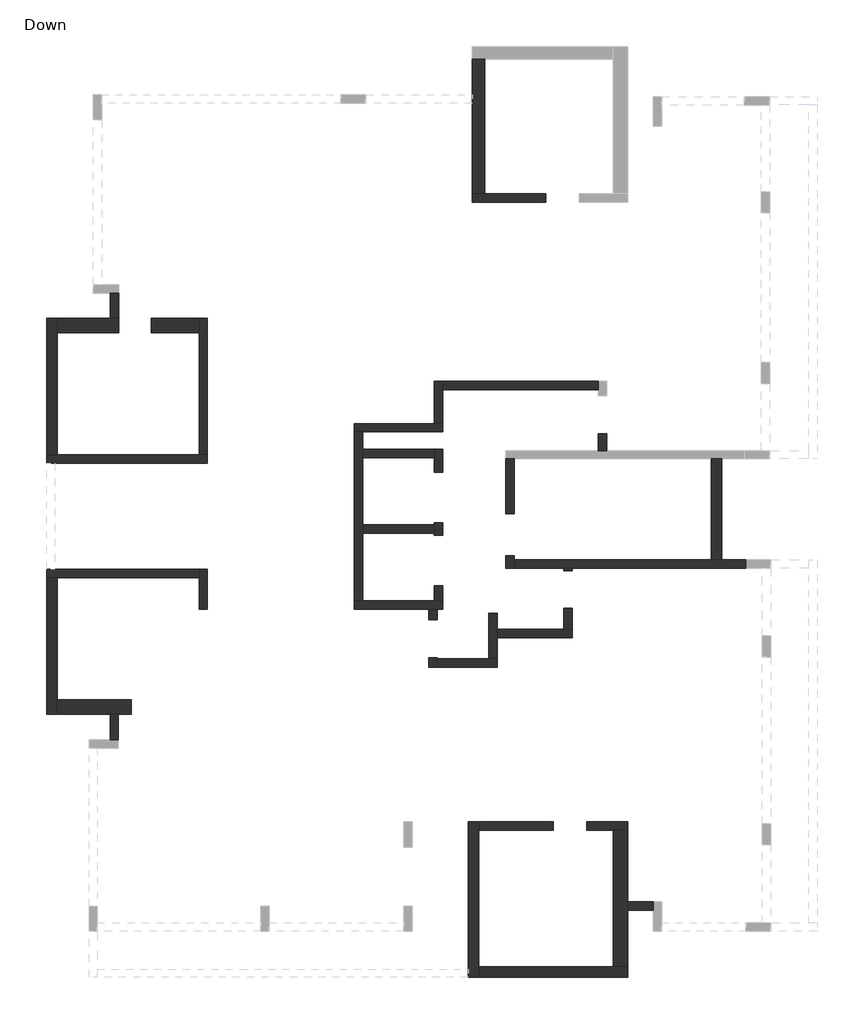
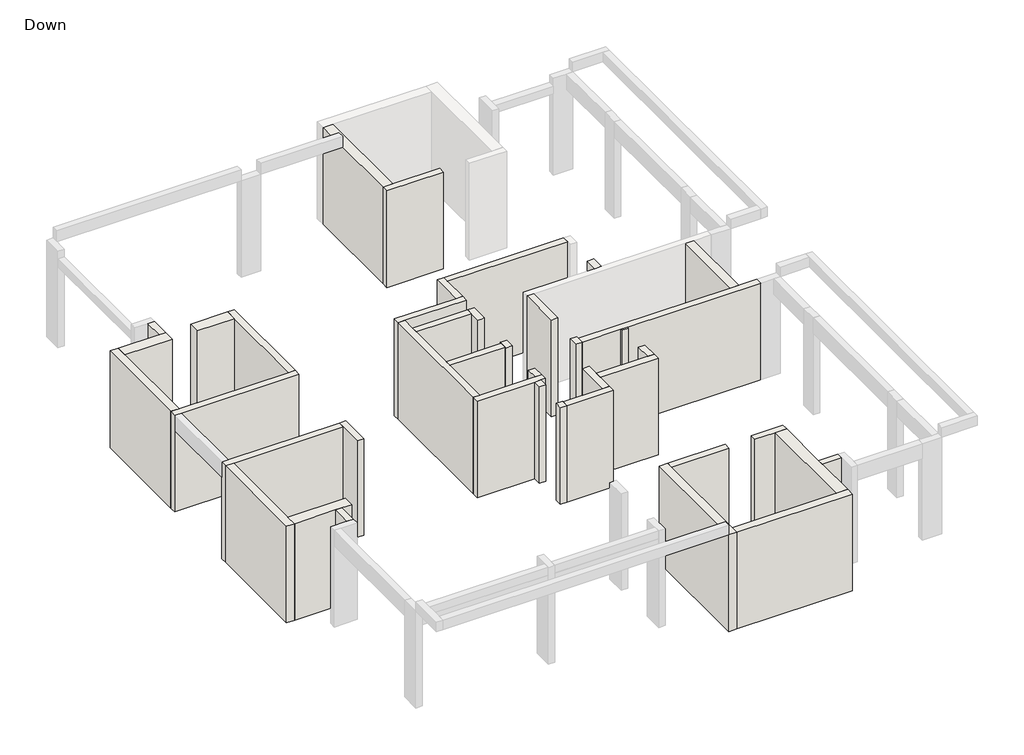
# One storey, part 1 of 2: 41 walls.
"""IFC4 building model written with IfcOpenShell, lengths in millimetres."""

from ifc_helpers import new_model, si_unit, origin, origin_with_axes, place, context, project, spatial, polyline, outline, extrude, faceted_brep, element, save

model = new_model("IFC4")

# Units and contexts
model_context = context("Model", 3, world=origin())
ifc_project = project(units=[si_unit("LENGTHUNIT", "METRE", prefix="MILLI")], contexts=[model_context])

# Site, building, storey
site = spatial("IfcSite", under=ifc_project)
building = spatial("IfcBuilding", under=site)
storey = spatial("IfcBuildingStorey", under=building, Name="Down", Elevation=0.0)

# Walls
placement = place(None, origin())
element("IfcWall", 1, ObjectType="20", at=placement, inside=storey, context=model_context, shape_type="Brep", body=[
    faceted_brep([(-7842.7593383, -3416.4704639, 0.0), (-7842.7593383, -2465.8036059, 0.0), (-7842.7593383, -2465.8036059, 2900.0), (-7842.7593383, -2465.8036059, 3150.0), (-7842.7593383, -3416.4704639, 3150.0), (-7842.7593383, -3416.4704639, 2900.0), (-8042.7593383, -3416.4704639, 0.0), (-8042.7593383, -3416.4704639, 2900.0), (-8042.7593383, -3416.4704639, 3150.0), (-8042.7593383, -2665.8036059, 3150.0), (-8042.7593383, -2465.8036059, 3150.0), (-8042.7593383, -2465.8036059, 0.0), (-8042.7593383, -2665.8036059, 0.0)], [[[0, 1, 2, 3, 4, 5]], [[6, 7, 8, 9, 10, 11, 12]], [[1, 0, 6, 12, 11]], [[4, 3, 10, 9, 8]], [[0, 5, 4, 8, 7, 6]], [[3, 2, 1, 11, 10]]]),
])
element("IfcWall", 2, ObjectType="20", at=placement, inside=storey, context=model_context, shape_type="Brep", body=[
    faceted_brep([(-8042.7593383, -2465.8036059, 0.0), (-11667.5737279, -2465.8036059, 0.0), (-11667.5737279, -2465.8036059, 3150.0), (-11467.5737279, -2465.8036059, 3150.0), (-8042.7593383, -2465.8036059, 3150.0), (-8042.7593383, -2665.8036059, 0.0), (-8042.7593383, -2665.8036059, 2900.0), (-8042.7593383, -2665.8036059, 3150.0), (-11417.5737279, -2665.8036059, 3150.0), (-11667.5737279, -2665.8036059, 3150.0), (-11667.5737279, -2665.8036059, 0.0), (-11417.5737279, -2665.8036059, 0.0)], [[[0, 1, 2, 3, 4]], [[5, 6, 7, 8, 9, 10, 11]], [[1, 0, 5, 11, 10]], [[4, 3, 2, 9, 8, 7]], [[0, 4, 7, 6, 5]], [[2, 1, 10, 9]]]),
])
element("IfcWall", 3, ObjectType="20", at=placement, inside=storey, context=model_context, shape_type="Brep", body=[
    faceted_brep([(-10157.6225223, -5916.9995493, 0.0), (-10157.6225223, -6521.9995493, 0.0), (-10157.6225223, -6521.9995493, 3150.0), (-10157.6225223, -5916.9995493, 3150.0), (-9957.6225223, -5916.9995493, 0.0), (-9957.6225223, -5916.9995493, 2900.0), (-9957.6225223, -5916.9995493, 3150.0), (-9957.6225223, -6521.9995493, 3150.0), (-9957.6225223, -6521.9995493, 0.0)], [[[0, 1, 2, 3]], [[4, 5, 6, 7, 8]], [[1, 0, 4, 8]], [[2, 1, 8, 7]], [[3, 2, 7, 6]], [[0, 3, 6, 5, 4]]]),
])
element("IfcWall", 4, ObjectType="20", at=placement, inside=storey, context=model_context, shape_type="Brep", body=[
    faceted_brep([(-11667.5737279, 47.4292682, 0.0), (-7841.6160164, 47.4292682, 0.0), (-7841.6160164, 47.4292682, 2900.0), (-7841.6160164, 47.4292682, 3150.0), (-11467.5737279, 47.4292682, 3150.0), (-11667.5737279, 47.4292682, 3150.0), (-11667.5737279, 247.4292682, 0.0), (-11667.5737279, 247.4292682, 3150.0), (-11417.5737279, 247.4292682, 3150.0), (-8041.6160164, 247.4292682, 3150.0), (-7841.6160164, 247.4292682, 3150.0), (-7841.6160164, 247.4292682, 0.0), (-8041.6160164, 247.4292682, 0.0), (-11417.5737279, 247.4292682, 0.0)], [[[0, 1, 2, 3, 4, 5]], [[6, 7, 8, 9, 10, 11, 12, 13]], [[1, 0, 6, 13, 12, 11]], [[5, 4, 3, 10, 9, 8, 7]], [[3, 2, 1, 11, 10]], [[0, 5, 7, 6]]]),
])
element("IfcWall", 5, ObjectType="20", at=placement, inside=storey, context=model_context, shape_type="Brep", body=[
    faceted_brep([(-7841.6160164, 247.4292682, 0.0), (-7841.6160164, 3498.6252115, 0.0), (-7841.6160164, 3498.6252115, 2900.0), (-7841.6160164, 3498.6252115, 3150.0), (-7841.6160164, 247.4292682, 3150.0), (-8041.6160164, 247.4292682, 0.0), (-8041.6160164, 247.4292682, 2900.0), (-8041.6160164, 247.4292682, 3150.0), (-8041.6160164, 3148.6252115, 3150.0), (-8041.6160164, 3498.6252115, 3150.0), (-8041.6160164, 3498.6252115, 0.0), (-8041.6160164, 3148.6252115, 0.0)], [[[0, 1, 2, 3, 4]], [[5, 6, 7, 8, 9, 10, 11]], [[1, 0, 5, 11, 10]], [[4, 3, 9, 8, 7]], [[0, 4, 7, 6, 5]], [[3, 2, 1, 10, 9]]]),
])
element("IfcWall", 6, ObjectType="20", at=placement, inside=storey, context=model_context, shape_type="Brep", body=[
    faceted_brep([(-4348.0741106, -3416.4704639, 0.0), (-2578.9868545, -3416.4704639, 0.0), (-2378.9868545, -3416.4704639, 0.0), (-2247.7143708, -3416.4704639, 0.0), (-2247.7143708, -3416.4704639, 2900.0), (-2247.7143708, -3416.4704639, 3150.0), (-2378.9868545, -3416.4704639, 3150.0), (-2578.9868545, -3416.4704639, 3150.0), (-4348.0741106, -3416.4704639, 3150.0), (-4348.0741106, -3416.4704639, 2900.0), (-4348.0741106, -3216.4704639, 0.0), (-4348.0741106, -3216.4704639, 3150.0), (-4148.0741106, -3216.4704639, 3150.0), (-2447.7143708, -3216.4704639, 3150.0), (-2247.7143708, -3216.4704639, 3150.0), (-2247.7143708, -3216.4704639, 0.0), (-2447.7143708, -3216.4704639, 0.0), (-4148.0741106, -3216.4704639, 0.0)], [[[0, 1, 2, 3, 4, 5, 6, 7, 8, 9]], [[10, 11, 12, 13, 14, 15, 16, 17]], [[3, 2, 1, 0, 10, 17, 16, 15]], [[8, 7, 6, 5, 14, 13, 12, 11]], [[5, 4, 3, 15, 14]], [[0, 9, 8, 11, 10]]]),
])
element("IfcWall", 7, ObjectType="20", at=placement, inside=storey, context=model_context, shape_type="Brep", body=[
    faceted_brep([(-2247.7143708, -3216.4704639, 0.0), (-2247.7143708, -2865.9729515, 0.0), (-2247.7143708, -2865.9729515, 2900.0), (-2247.7143708, -2865.9729515, 3150.0), (-2247.7143708, -3216.4704639, 3150.0), (-2447.7143708, -3216.4704639, 0.0), (-2447.7143708, -3216.4704639, 3150.0), (-2447.7143708, -2865.9729515, 3150.0), (-2447.7143708, -2865.9729515, 0.0), (-2347.7143708, -2865.9729515, 3150.0)], [[[0, 1, 2, 3, 4]], [[5, 6, 7, 8]], [[1, 0, 5, 8]], [[3, 2, 1, 8, 7, 9]], [[4, 3, 9, 7, 6]], [[0, 4, 6, 5]]]),
])
element("IfcWall", 8, ObjectType="20", at=placement, inside=storey, context=model_context, shape_type="Brep", body=[
    faceted_brep([(-2247.7143708, -1665.4649148, 0.0), (-2247.7143708, -1366.9258792, 0.0), (-2247.7143708, -1366.9258792, 2900.0), (-2247.7143708, -1366.9258792, 3150.0), (-2247.7143708, -1665.4649148, 3150.0), (-2247.7143708, -1665.4649148, 2900.0), (-2447.7143708, -1665.4649148, 0.0), (-2447.7143708, -1665.4649148, 3150.0), (-2447.7143708, -1616.7670579, 3150.0), (-2447.7143708, -1416.7670579, 3150.0), (-2447.7143708, -1366.9258792, 3150.0), (-2447.7143708, -1366.9258792, 0.0), (-2447.7143708, -1416.7670579, 0.0), (-2447.7143708, -1616.7670579, 0.0), (-2347.7143708, -1366.9258792, 3150.0), (-2347.7143708, -1665.4649148, 3150.0)], [[[0, 1, 2, 3, 4, 5]], [[6, 7, 8, 9, 10, 11, 12, 13]], [[1, 0, 6, 13, 12, 11]], [[3, 2, 1, 11, 10, 14]], [[4, 3, 14, 10, 9, 8, 7, 15]], [[0, 5, 4, 15, 7, 6]]]),
])
element("IfcWall", 9, ObjectType="20", at=placement, inside=storey, context=model_context, shape_type="SweptSolid", body=[
    extrude(outline(polyline([(-4148.0741106, -1416.7670579), (-2447.7143708, -1416.7670579), (-2447.7143708, -1616.7670579), (-4148.0741106, -1616.7670579), (-4148.0741106, -1416.7670579)])), origin_with_axes(), (0.0, 0.0, 1.0), 3150.0),
])
element("IfcWall", 10, ObjectType="20", at=placement, inside=storey, context=model_context, shape_type="Brep", body=[
    faceted_brep([(-4348.0741106, 794.07967, 0.0), (-4348.0741106, -3216.4704639, 0.0), (-4348.0741106, -3216.4704639, 3150.0), (-4348.0741106, 47.4292682, 3150.0), (-4348.0741106, 794.07967, 3150.0), (-4148.0741106, 794.07967, 0.0), (-4148.0741106, 794.07967, 2900.0), (-4148.0741106, 794.07967, 3150.0), (-4148.0741106, 384.07967, 3150.0), (-4148.0741106, 184.07967, 3150.0), (-4148.0741106, -1416.7670579, 3150.0), (-4148.0741106, -1616.7670579, 3150.0), (-4148.0741106, -3216.4704639, 3150.0), (-4148.0741106, -3216.4704639, 0.0), (-4148.0741106, -1616.7670579, 0.0), (-4148.0741106, -1416.7670579, 0.0), (-4148.0741106, 184.07967, 0.0), (-4148.0741106, 384.07967, 0.0)], [[[0, 1, 2, 3, 4]], [[5, 6, 7, 8, 9, 10, 11, 12, 13, 14, 15, 16, 17]], [[1, 0, 5, 17, 16, 15, 14, 13]], [[4, 3, 2, 12, 11, 10, 9, 8, 7]], [[2, 1, 13, 12]], [[0, 4, 7, 6, 5]]]),
])
element("IfcWall", 11, ObjectType="20", at=placement, inside=storey, context=model_context, shape_type="Brep", body=[
    faceted_brep([(-2247.7143708, -166.4178424, 0.0), (-2247.7143708, 384.07967, 0.0), (-2247.7143708, 384.07967, 2900.0), (-2247.7143708, 384.07967, 3150.0), (-2247.7143708, -166.4178424, 3150.0), (-2247.7143708, -166.4178424, 2900.0), (-2447.7143708, -166.4178424, 0.0), (-2447.7143708, -166.4178424, 3150.0), (-2447.7143708, 184.07967, 3150.0), (-2447.7143708, 384.07967, 3150.0), (-2447.7143708, 384.07967, 0.0), (-2447.7143708, 184.07967, 0.0), (-2347.7143708, -166.4178424, 3150.0)], [[[0, 1, 2, 3, 4, 5]], [[6, 7, 8, 9, 10, 11]], [[1, 0, 6, 11, 10]], [[4, 3, 9, 8, 7, 12]], [[0, 5, 4, 12, 7, 6]], [[3, 2, 1, 10, 9]]]),
])
element("IfcWall", 12, ObjectType="20", at=placement, inside=storey, context=model_context, shape_type="Brep", body=[
    faceted_brep([(-2447.7143708, 384.07967, 0.0), (-4148.0741106, 384.07967, 0.0), (-4148.0741106, 384.07967, 2900.0), (-4148.0741106, 384.07967, 3150.0), (-2447.7143708, 384.07967, 3150.0), (-2447.7143708, 184.07967, 0.0), (-2447.7143708, 184.07967, 3150.0), (-4148.0741106, 184.07967, 3150.0), (-4148.0741106, 184.07967, 0.0)], [[[0, 1, 2, 3, 4]], [[5, 6, 7, 8]], [[1, 0, 5, 8]], [[4, 3, 7, 6]], [[0, 4, 6, 5]], [[3, 2, 1, 8, 7]]]),
])
element("IfcWall", 13, ObjectType="20", at=placement, inside=storey, context=model_context, shape_type="Brep", body=[
    faceted_brep([(-4348.0741106, 794.07967, 0.0), (-4148.0741106, 794.07967, 0.0), (-2249.8316689, 794.07967, 0.0), (-2249.8316689, 794.07967, 2900.0), (-2249.8316689, 794.07967, 3150.0), (-4148.0741106, 794.07967, 3150.0), (-4348.0741106, 794.07967, 3150.0), (-4348.0741106, 994.07967, 0.0), (-4348.0741106, 994.07967, 2900.0), (-4348.0741106, 994.07967, 3150.0), (-2449.8316689, 994.07967, 3150.0), (-2249.8316689, 994.07967, 3150.0), (-2249.8316689, 994.07967, 0.0), (-2449.8316689, 994.07967, 0.0)], [[[0, 1, 2, 3, 4, 5, 6]], [[7, 8, 9, 10, 11, 12, 13]], [[2, 1, 0, 7, 13, 12]], [[6, 5, 4, 11, 10, 9]], [[4, 3, 2, 12, 11]], [[0, 6, 9, 8, 7]]]),
])
element("IfcWall", 14, ObjectType="20", at=placement, inside=storey, context=model_context, shape_type="Brep", body=[
    faceted_brep([(-2249.8316689, 994.07967, 0.0), (-2249.8316689, 1803.8127355, 0.0), (-2249.8316689, 2003.8127355, 0.0), (-2249.8316689, 2003.8127355, 3150.0), (-2249.8316689, 1803.8127355, 3150.0), (-2249.8316689, 994.07967, 3150.0), (-2449.8316689, 994.07967, 0.0), (-2449.8316689, 994.07967, 2900.0), (-2449.8316689, 994.07967, 3150.0), (-2449.8316689, 2003.8127355, 3150.0), (-2449.8316689, 2003.8127355, 2900.0), (-2449.8316689, 2003.8127355, 0.0)], [[[0, 1, 2, 3, 4, 5]], [[6, 7, 8, 9, 10, 11]], [[2, 1, 0, 6, 11]], [[5, 4, 3, 9, 8]], [[0, 5, 8, 7, 6]], [[3, 2, 11, 10, 9]]]),
])
element("IfcWall", 15, ObjectType="20", at=placement, inside=storey, context=model_context, shape_type="Brep", body=[
    faceted_brep([(-2249.8316689, 1803.8127355, 0.0), (1452.348775, 1803.8127355, 0.0), (1452.348775, 1803.8127355, 2900.0), (1452.348775, 1803.8127355, 3150.0), (-2249.8316689, 1803.8127355, 3150.0), (-2249.8316689, 1803.8127355, 2900.0), (-2249.8316689, 2003.8127355, 0.0), (-2249.8316689, 2003.8127355, 3150.0), (1452.348775, 2003.8127355, 3150.0), (1452.348775, 2003.8127355, 0.0)], [[[0, 1, 2, 3, 4, 5]], [[6, 7, 8, 9]], [[1, 0, 6, 9]], [[4, 3, 8, 7]], [[0, 5, 4, 7, 6]], [[3, 2, 1, 9, 8]]]),
])
element("IfcWall", 16, ObjectType="20", at=placement, inside=storey, context=model_context, shape_type="Brep", body=[
    faceted_brep([(1452.348775, 750.3722456, 0.0), (1452.348775, 352.3201981, 0.0), (1452.348775, 352.3201981, 2900.0), (1452.348775, 352.3201981, 3150.0), (1452.348775, 750.3722456, 3150.0), (1452.348775, 750.3722456, 2900.0), (1652.348775, 750.3722456, 0.0), (1652.348775, 750.3722456, 2900.0), (1652.348775, 750.3722456, 3150.0), (1652.348775, 352.3201981, 3150.0), (1652.348775, 352.3201981, 2900.0), (1652.348775, 352.3201981, 0.0), (1552.348775, 750.3722456, 3150.0)], [[[0, 1, 2, 3, 4, 5]], [[6, 7, 8, 9, 10, 11]], [[1, 0, 6, 11]], [[4, 3, 9, 8, 12]], [[0, 5, 4, 12, 8, 7, 6]], [[3, 2, 1, 11, 10, 9]]]),
])
element("IfcWall", 17, ObjectType="20", at=placement, inside=storey, context=model_context, shape_type="Brep", body=[
    faceted_brep([(-748.6672985, 152.3201981, 0.0), (-748.6672985, -1148.8441723, 0.0), (-748.6672985, -1148.8441723, 2900.0), (-748.6672985, -1148.8441723, 3150.0), (-748.6672985, 152.3201981, 3150.0), (-548.6672985, 152.3201981, 0.0), (-548.6672985, 152.3201981, 3150.0), (-548.6672985, -1148.8441723, 3150.0), (-548.6672985, -1148.8441723, 2900.0), (-548.6672985, -1148.8441723, 0.0)], [[[0, 1, 2, 3, 4]], [[5, 6, 7, 8, 9]], [[1, 0, 5, 9]], [[3, 2, 1, 9, 8, 7]], [[4, 3, 7, 6]], [[0, 4, 6, 5]]]),
])
element("IfcWall", 18, ObjectType="20", at=placement, inside=storey, context=model_context, shape_type="Brep", body=[
    faceted_brep([(-748.6672985, -2148.2088872, 0.0), (-748.6672985, -2446.7479228, 0.0), (-748.6672985, -2446.7479228, 2900.0), (-748.6672985, -2446.7479228, 3150.0), (-748.6672985, -2148.2088872, 3150.0), (-748.6672985, -2148.2088872, 2900.0), (-548.6672985, -2148.2088872, 0.0), (-548.6672985, -2148.2088872, 2900.0), (-548.6672985, -2148.2088872, 3150.0), (-548.6672985, -2246.7479228, 3150.0), (-548.6672985, -2446.7479228, 3150.0), (-548.6672985, -2446.7479228, 0.0), (-548.6672985, -2246.7479228, 0.0)], [[[0, 1, 2, 3, 4, 5]], [[6, 7, 8, 9, 10, 11, 12]], [[1, 0, 6, 12, 11]], [[4, 3, 10, 9, 8]], [[0, 5, 4, 8, 7, 6]], [[3, 2, 1, 11, 10]]]),
])
element("IfcWall", 19, ObjectType="20", at=placement, inside=storey, context=model_context, shape_type="Brep", body=[
    faceted_brep([(-548.6672985, -2446.7479228, 0.0), (633.928377, -2446.7479228, 0.0), (833.928377, -2446.7479228, 0.0), (4951.7310336, -2446.7479228, 0.0), (4951.7310336, -2446.7479228, 3150.0), (833.928377, -2446.7479228, 3150.0), (633.928377, -2446.7479228, 3150.0), (-548.6672985, -2446.7479228, 3150.0), (-548.6672985, -2246.7479228, 0.0), (-548.6672985, -2246.7479228, 3150.0), (4133.663356, -2246.7479228, 3150.0), (4383.663356, -2246.7479228, 3150.0), (4951.7310336, -2246.7479228, 3150.0), (4951.7310336, -2246.7479228, 0.0), (4383.663356, -2246.7479228, 0.0), (4133.663356, -2246.7479228, 0.0)], [[[0, 1, 2, 3, 4, 5, 6, 7]], [[8, 9, 10, 11, 12, 13, 14, 15]], [[3, 2, 1, 0, 8, 15, 14, 13]], [[4, 3, 13, 12]], [[7, 6, 5, 4, 12, 11, 10, 9]], [[0, 7, 9, 8]]]),
])
element("IfcWall", 20, ObjectType="20", at=placement, inside=storey, context=model_context, shape_type="Brep", body=[
    faceted_brep([(-1396.4017034, -8672.5783859, 0.0), (379.852602, -8672.5783859, 0.0), (379.852602, -8672.5783859, 2900.0), (379.852602, -8672.5783859, 3150.0), (-1396.4017034, -8672.5783859, 3150.0), (-1396.4017034, -8672.5783859, 2900.0), (-1396.4017034, -8472.5783859, 0.0), (-1396.4017034, -8472.5783859, 3150.0), (379.852602, -8472.5783859, 3150.0), (379.852602, -8472.5783859, 2900.0), (379.852602, -8472.5783859, 0.0)], [[[0, 1, 2, 3, 4, 5]], [[6, 7, 8, 9, 10]], [[1, 0, 6, 10]], [[3, 2, 1, 10, 9, 8]], [[4, 3, 8, 7]], [[0, 5, 4, 7, 6]]]),
])
element("IfcWall", 21, ObjectType="20", at=placement, inside=storey, context=model_context, shape_type="Brep", body=[
    faceted_brep([(1180.1912932, -8672.5783859, 0.0), (1805.1912932, -8672.5783859, 0.0), (2155.1912932, -8672.5783859, 0.0), (2155.1912932, -8672.5783859, 3150.0), (1805.1912932, -8672.5783859, 3150.0), (1180.1912932, -8672.5783859, 3150.0), (1180.1912932, -8672.5783859, 2900.0), (1180.1912932, -8472.5783859, 0.0), (1180.1912932, -8472.5783859, 2900.0), (1180.1912932, -8472.5783859, 3150.0), (2155.1912932, -8472.5783859, 3150.0), (2155.1912932, -8472.5783859, 2900.0), (2155.1912932, -8472.5783859, 0.0)], [[[0, 1, 2, 3, 4, 5, 6]], [[7, 8, 9, 10, 11, 12]], [[2, 1, 0, 7, 12]], [[5, 4, 3, 10, 9]], [[0, 6, 5, 9, 8, 7]], [[3, 2, 12, 11, 10]]]),
])
element("IfcWall", 22, ObjectType="20", at=placement, inside=storey, context=model_context, shape_type="Brep", body=[
    faceted_brep([(2753.3437999, -10374.7377812, 0.0), (2155.1912932, -10374.7377812, 0.0), (2155.1912932, -10374.7377812, 2900.0), (2155.1912932, -10374.7377812, 3150.0), (2753.3437999, -10374.7377812, 3150.0), (2753.3437999, -10574.7377812, 0.0), (2753.3437999, -10574.7377812, 3150.0), (2155.1912932, -10574.7377812, 3150.0), (2155.1912932, -10574.7377812, 0.0)], [[[0, 1, 2, 3, 4]], [[5, 6, 7, 8]], [[1, 0, 5, 8]], [[4, 3, 7, 6]], [[0, 4, 6, 5]], [[3, 2, 1, 8, 7]]]),
])
element("IfcWall", 23, ObjectType="20", at=placement, inside=storey, context=model_context, shape_type="Brep", body=[
    faceted_brep([(-2578.9868545, -3416.4704639, 0.0), (-2578.9868545, -3670.5462389, 0.0), (-2578.9868545, -3670.5462389, 2900.0), (-2578.9868545, -3670.5462389, 3150.0), (-2578.9868545, -3416.4704639, 3150.0), (-2578.9868545, -3416.4704639, 2900.0), (-2378.9868545, -3416.4704639, 0.0), (-2378.9868545, -3416.4704639, 2900.0), (-2378.9868545, -3416.4704639, 3150.0), (-2378.9868545, -3670.5462389, 3150.0), (-2378.9868545, -3670.5462389, 2900.0), (-2378.9868545, -3670.5462389, 0.0)], [[[0, 1, 2, 3, 4, 5]], [[6, 7, 8, 9, 10, 11]], [[1, 0, 6, 11]], [[3, 2, 1, 11, 10, 9]], [[4, 3, 9, 8]], [[0, 5, 4, 8, 7, 6]]]),
])
element("IfcWall", 24, ObjectType="20", at=placement, inside=storey, context=model_context, shape_type="Brep", body=[
    faceted_brep([(-2578.9868545, -4570.3979419, 0.0), (-2578.9868545, -4796.9488413, 0.0), (-2578.9868545, -4796.9488413, 2900.0), (-2578.9868545, -4796.9488413, 3150.0), (-2578.9868545, -4570.3979419, 3150.0), (-2578.9868545, -4570.3979419, 2900.0), (-2378.9868545, -4570.3979419, 0.0), (-2378.9868545, -4570.3979419, 2900.0), (-2378.9868545, -4570.3979419, 3150.0), (-2378.9868545, -4596.9488413, 3150.0), (-2378.9868545, -4796.9488413, 3150.0), (-2378.9868545, -4796.9488413, 0.0), (-2378.9868545, -4596.9488413, 0.0)], [[[0, 1, 2, 3, 4, 5]], [[6, 7, 8, 9, 10, 11, 12]], [[1, 0, 6, 12, 11]], [[4, 3, 10, 9, 8]], [[0, 5, 4, 8, 7, 6]], [[3, 2, 1, 11, 10]]]),
])
element("IfcWall", 25, ObjectType="20", at=placement, inside=storey, context=model_context, shape_type="Brep", body=[
    faceted_brep([(-2378.9868545, -4796.9488413, 0.0), (-951.9279184, -4796.9488413, 0.0), (-951.9279184, -4796.9488413, 2900.0), (-951.9279184, -4796.9488413, 3150.0), (-2378.9868545, -4796.9488413, 3150.0), (-2378.9868545, -4596.9488413, 0.0), (-2378.9868545, -4596.9488413, 2900.0), (-2378.9868545, -4596.9488413, 3150.0), (-1151.9279184, -4596.9488413, 3150.0), (-951.9279184, -4596.9488413, 3150.0), (-951.9279184, -4596.9488413, 0.0), (-1151.9279184, -4596.9488413, 0.0)], [[[0, 1, 2, 3, 4]], [[5, 6, 7, 8, 9, 10, 11]], [[1, 0, 5, 11, 10]], [[4, 3, 9, 8, 7]], [[0, 4, 7, 6, 5]], [[3, 2, 1, 10, 9]]]),
])
element("IfcWall", 26, ObjectType="20", at=placement, inside=storey, context=model_context, shape_type="Brep", body=[
    faceted_brep([(-951.9279184, -4596.9488413, 0.0), (-951.9279184, -4098.2404601, 0.0), (-951.9279184, -3898.2404601, 0.0), (-951.9279184, -3515.9834758, 0.0), (-951.9279184, -3515.9834758, 2900.0), (-951.9279184, -3515.9834758, 3150.0), (-951.9279184, -3898.2404601, 3150.0), (-951.9279184, -4098.2404601, 3150.0), (-951.9279184, -4596.9488413, 3150.0), (-1151.9279184, -4596.9488413, 0.0), (-1151.9279184, -4596.9488413, 2900.0), (-1151.9279184, -4596.9488413, 3150.0), (-1151.9279184, -3515.9834758, 3150.0), (-1151.9279184, -3515.9834758, 2900.0), (-1151.9279184, -3515.9834758, 0.0)], [[[0, 1, 2, 3, 4, 5, 6, 7, 8]], [[9, 10, 11, 12, 13, 14]], [[3, 2, 1, 0, 9, 14]], [[5, 4, 3, 14, 13, 12]], [[8, 7, 6, 5, 12, 11]], [[0, 8, 11, 10, 9]]]),
])
element("IfcWall", 27, ObjectType="20", at=placement, inside=storey, context=model_context, shape_type="Brep", body=[
    faceted_brep([(-951.9279184, -4098.2404601, 0.0), (833.928377, -4098.2404601, 0.0), (833.928377, -4098.2404601, 2900.0), (833.928377, -4098.2404601, 3150.0), (-951.9279184, -4098.2404601, 3150.0), (-951.9279184, -4098.2404601, 2900.0), (-951.9279184, -3898.2404601, 0.0), (-951.9279184, -3898.2404601, 2900.0), (-951.9279184, -3898.2404601, 3150.0), (633.928377, -3898.2404601, 3150.0), (833.928377, -3898.2404601, 3150.0), (833.928377, -3898.2404601, 0.0), (633.928377, -3898.2404601, 0.0)], [[[0, 1, 2, 3, 4, 5]], [[6, 7, 8, 9, 10, 11, 12]], [[1, 0, 6, 12, 11]], [[4, 3, 10, 9, 8]], [[0, 5, 4, 8, 7, 6]], [[3, 2, 1, 11, 10]]]),
])
element("IfcWall", 28, ObjectType="20", at=placement, inside=storey, context=model_context, shape_type="Brep", body=[
    faceted_brep([(833.928377, -3898.2404601, 0.0), (833.928377, -3399.5320789, 0.0), (833.928377, -3399.5320789, 2900.0), (833.928377, -3399.5320789, 3150.0), (833.928377, -3898.2404601, 3150.0), (633.928377, -3898.2404601, 0.0), (633.928377, -3898.2404601, 2900.0), (633.928377, -3898.2404601, 3150.0), (633.928377, -3399.5320789, 3150.0), (633.928377, -3399.5320789, 2900.0), (633.928377, -3399.5320789, 0.0)], [[[0, 1, 2, 3, 4]], [[5, 6, 7, 8, 9, 10]], [[1, 0, 5, 10]], [[3, 2, 1, 10, 9, 8]], [[4, 3, 8, 7]], [[0, 4, 7, 6, 5]]]),
])
element("IfcWall", 29, ObjectType="20", at=placement, inside=storey, context=model_context, shape_type="Brep", body=[
    faceted_brep([(833.928377, -2499.6803759, 0.0), (833.928377, -2446.7479228, 0.0), (833.928377, -2446.7479228, 2900.0), (833.928377, -2446.7479228, 3150.0), (833.928377, -2499.6803759, 3150.0), (833.928377, -2499.6803759, 2900.0), (633.928377, -2499.6803759, 0.0), (633.928377, -2499.6803759, 2900.0), (633.928377, -2499.6803759, 3150.0), (633.928377, -2446.7479228, 3150.0), (633.928377, -2446.7479228, 2900.0), (633.928377, -2446.7479228, 0.0)], [[[0, 1, 2, 3, 4, 5]], [[6, 7, 8, 9, 10, 11]], [[1, 0, 6, 11]], [[4, 3, 9, 8]], [[0, 5, 4, 8, 7, 6]], [[3, 2, 1, 11, 10, 9]]]),
])
element("IfcWall", 30, ObjectType="20", at=placement, inside=storey, context=model_context, shape_type="Brep", body=[
    faceted_brep([(-1546.8886915, 6257.4646681, 0.0), (199.8822614, 6257.4646681, 0.0), (199.8822614, 6257.4646681, 2900.0), (199.8822614, 6257.4646681, 3150.0), (-1546.8886915, 6257.4646681, 3150.0), (-1546.8886915, 6257.4646681, 2900.0), (-1546.8886915, 6457.4646681, 0.0), (-1546.8886915, 6457.4646681, 3150.0), (-1246.8886915, 6457.4646681, 3150.0), (199.8822614, 6457.4646681, 3150.0), (199.8822614, 6457.4646681, 2900.0), (199.8822614, 6457.4646681, 0.0), (-1246.8886915, 6457.4646681, 0.0)], [[[0, 1, 2, 3, 4, 5]], [[6, 7, 8, 9, 10, 11, 12]], [[1, 0, 6, 12, 11]], [[3, 2, 1, 11, 10, 9]], [[4, 3, 9, 8, 7]], [[0, 5, 4, 7, 6]]]),
])
element("IfcWall", 31, ObjectType="20", at=placement, inside=storey, context=model_context, shape_type="SweptSolid", body=[
    extrude(outline(polyline([(-9955.8228668, 4097.8205808), (-9955.8228668, 3498.6252115), (-10155.8228668, 3498.6252115), (-10155.8228668, 4097.8205808), (-9955.8228668, 4097.8205808)])), origin_with_axes(), (0.0, 0.0, 1.0), 3150.0),
])
element("IfcWall", 32, ObjectType="25", at=placement, inside=storey, context=model_context, shape_type="Brep", body=[
    faceted_brep([(-11667.5737279, -2665.8036059, 0.0), (-11667.5737279, -5916.9995493, 0.0), (-11667.5737279, -5916.9995493, 3150.0), (-11667.5737279, -2665.8036059, 3150.0), (-11417.5737279, -2665.8036059, 0.0), (-11417.5737279, -2665.8036059, 2900.0), (-11417.5737279, -2665.8036059, 3150.0), (-11417.5737279, -5566.9995493, 3150.0), (-11417.5737279, -5916.9995493, 3150.0), (-11417.5737279, -5916.9995493, 0.0), (-11417.5737279, -5566.9995493, 0.0)], [[[0, 1, 2, 3]], [[4, 5, 6, 7, 8, 9, 10]], [[1, 0, 4, 10, 9]], [[3, 2, 8, 7, 6]], [[0, 3, 6, 5, 4]], [[2, 1, 9, 8]]]),
])
element("IfcWall", 33, ObjectType="25", at=placement, inside=storey, context=model_context, shape_type="Brep", body=[
    faceted_brep([(-11417.5737279, 247.4292682, 0.0), (-11417.5737279, 3148.6252115, 0.0), (-11417.5737279, 3498.6252115, 0.0), (-11417.5737279, 3498.6252115, 3150.0), (-11417.5737279, 3148.6252115, 3150.0), (-11417.5737279, 247.4292682, 3150.0), (-11417.5737279, 247.4292682, 2900.0), (-11667.5737279, 247.4292682, 0.0), (-11667.5737279, 247.4292682, 3150.0), (-11667.5737279, 3498.6252115, 3150.0), (-11667.5737279, 3498.6252115, 0.0)], [[[0, 1, 2, 3, 4, 5, 6]], [[7, 8, 9, 10]], [[2, 1, 0, 7, 10]], [[5, 4, 3, 9, 8]], [[3, 2, 10, 9]], [[0, 6, 5, 8, 7]]]),
])
element("IfcWall", 34, ObjectType="25", at=placement, inside=storey, context=model_context, shape_type="SweptSolid", body=[
    extrude(outline(polyline([(4383.663356, 152.3201981), (4383.663356, -2246.7479228), (4133.663356, -2246.7479228), (4133.663356, 152.3201981), (4383.663356, 152.3201981)])), origin_with_axes(), (0.0, 0.0, 1.0), 3150.0),
])
element("IfcWall", 35, ObjectType="25", at=placement, inside=storey, context=model_context, shape_type="Brep", body=[
    faceted_brep([(-1646.4017034, -8472.5783859, 0.0), (-1646.4017034, -12173.6155079, 0.0), (-1646.4017034, -12173.6155079, 2900.0), (-1646.4017034, -12173.6155079, 3150.0), (-1646.4017034, -11075.5031849, 3150.0), (-1646.4017034, -8472.5783859, 3150.0), (-1646.4017034, -8472.5783859, 2900.0), (-1396.4017034, -8472.5783859, 0.0), (-1396.4017034, -8472.5783859, 3150.0), (-1396.4017034, -8672.5783859, 3150.0), (-1396.4017034, -11923.6155079, 3150.0), (-1396.4017034, -12173.6155079, 3150.0), (-1396.4017034, -12173.6155079, 0.0), (-1396.4017034, -11923.6155079, 0.0), (-1396.4017034, -8672.5783859, 0.0)], [[[0, 1, 2, 3, 4, 5, 6]], [[7, 8, 9, 10, 11, 12, 13, 14]], [[1, 0, 7, 14, 13, 12]], [[5, 4, 3, 11, 10, 9, 8]], [[3, 2, 1, 12, 11]], [[0, 6, 5, 8, 7]]]),
])
element("IfcWall", 36, ObjectType="25", at=placement, inside=storey, context=model_context, shape_type="Brep", body=[
    faceted_brep([(-1396.4017034, -12173.6155079, 0.0), (2155.1912932, -12173.6155079, 0.0), (2155.1912932, -12173.6155079, 3150.0), (-1396.4017034, -12173.6155079, 3150.0), (-1396.4017034, -11923.6155079, 0.0), (-1396.4017034, -11923.6155079, 2900.0), (-1396.4017034, -11923.6155079, 3150.0), (1805.1912932, -11923.6155079, 3150.0), (2155.1912932, -11923.6155079, 3150.0), (2155.1912932, -11923.6155079, 0.0), (1805.1912932, -11923.6155079, 0.0)], [[[0, 1, 2, 3]], [[4, 5, 6, 7, 8, 9, 10]], [[1, 0, 4, 10, 9]], [[3, 2, 8, 7, 6]], [[0, 3, 6, 5, 4]], [[2, 1, 9, 8]]]),
])
element("IfcWall", 37, ObjectType="30", at=placement, inside=storey, context=model_context, shape_type="Brep", body=[
    faceted_brep([(-1546.8886915, 9657.4646681, 0.0), (-1546.8886915, 6457.4646681, 0.0), (-1546.8886915, 6457.4646681, 3150.0), (-1546.8886915, 8813.0435047, 3150.0), (-1546.8886915, 9657.4646681, 3150.0), (-1246.8886915, 9657.4646681, 0.0), (-1246.8886915, 9657.4646681, 2900.0), (-1246.8886915, 9657.4646681, 3150.0), (-1246.8886915, 6457.4646681, 3150.0), (-1246.8886915, 6457.4646681, 2900.0), (-1246.8886915, 6457.4646681, 0.0)], [[[0, 1, 2, 3, 4]], [[5, 6, 7, 8, 9, 10]], [[1, 0, 5, 10]], [[4, 3, 2, 8, 7]], [[2, 1, 10, 9, 8]], [[0, 4, 7, 6, 5]]]),
])
element("IfcWall", 38, ObjectType="35", at=placement, inside=storey, context=model_context, shape_type="Brep", body=[
    faceted_brep([(-11417.5737279, -5916.9995493, 0.0), (-10157.6225223, -5916.9995493, 0.0), (-9957.6225223, -5916.9995493, 0.0), (-9656.1405093, -5916.9995493, 0.0), (-9656.1405093, -5916.9995493, 2900.0), (-9656.1405093, -5916.9995493, 3150.0), (-9957.6225223, -5916.9995493, 3150.0), (-10157.6225223, -5916.9995493, 3150.0), (-11417.5737279, -5916.9995493, 3150.0), (-11417.5737279, -5566.9995493, 0.0), (-11417.5737279, -5566.9995493, 2900.0), (-11417.5737279, -5566.9995493, 3150.0), (-9656.1405093, -5566.9995493, 3150.0), (-9656.1405093, -5566.9995493, 2900.0), (-9656.1405093, -5566.9995493, 0.0)], [[[0, 1, 2, 3, 4, 5, 6, 7, 8]], [[9, 10, 11, 12, 13, 14]], [[3, 2, 1, 0, 9, 14]], [[5, 4, 3, 14, 13, 12]], [[8, 7, 6, 5, 12, 11]], [[0, 8, 11, 10, 9]]]),
])
element("IfcWall", 39, ObjectType="35", at=placement, inside=storey, context=model_context, shape_type="Brep", body=[
    faceted_brep([(-11417.5737279, 3148.6252115, 0.0), (-9955.8228668, 3148.6252115, 0.0), (-9955.8228668, 3148.6252115, 2900.0), (-9955.8228668, 3148.6252115, 3150.0), (-11417.5737279, 3148.6252115, 3150.0), (-11417.5737279, 3148.6252115, 2900.0), (-11417.5737279, 3498.6252115, 0.0), (-11417.5737279, 3498.6252115, 3150.0), (-10155.8228668, 3498.6252115, 3150.0), (-9955.8228668, 3498.6252115, 3150.0), (-9955.8228668, 3498.6252115, 0.0), (-10155.8228668, 3498.6252115, 0.0)], [[[0, 1, 2, 3, 4, 5]], [[6, 7, 8, 9, 10, 11]], [[1, 0, 6, 11, 10]], [[4, 3, 9, 8, 7]], [[0, 5, 4, 7, 6]], [[3, 2, 1, 10, 9]]]),
])
element("IfcWall", 40, ObjectType="35", at=placement, inside=storey, context=model_context, shape_type="Brep", body=[
    faceted_brep([(1805.1912932, -8672.5783859, 0.0), (1805.1912932, -11923.6155079, 0.0), (1805.1912932, -11923.6155079, 2900.0), (1805.1912932, -11923.6155079, 3150.0), (1805.1912932, -8672.5783859, 3150.0), (1805.1912932, -8672.5783859, 2900.0), (2155.1912932, -8672.5783859, 0.0), (2155.1912932, -8672.5783859, 3150.0), (2155.1912932, -10374.7377812, 3150.0), (2155.1912932, -10574.7377812, 3150.0), (2155.1912932, -11923.6155079, 3150.0), (2155.1912932, -11923.6155079, 0.0), (2155.1912932, -10574.7377812, 0.0), (2155.1912932, -10374.7377812, 0.0)], [[[0, 1, 2, 3, 4, 5]], [[6, 7, 8, 9, 10, 11, 12, 13]], [[1, 0, 6, 13, 12, 11]], [[4, 3, 10, 9, 8, 7]], [[3, 2, 1, 11, 10]], [[0, 5, 4, 7, 6]]]),
])
element("IfcWall", 41, ObjectType="35", at=placement, inside=storey, context=model_context, shape_type="Brep", body=[
    faceted_brep([(-8041.6160164, 3498.6252115, 0.0), (-9181.8657294, 3498.6252115, 0.0), (-9181.8657294, 3498.6252115, 2900.0), (-9181.8657294, 3498.6252115, 3150.0), (-8041.6160164, 3498.6252115, 3150.0), (-8041.6160164, 3148.6252115, 0.0), (-8041.6160164, 3148.6252115, 2900.0), (-8041.6160164, 3148.6252115, 3150.0), (-9181.8657294, 3148.6252115, 3150.0), (-9181.8657294, 3148.6252115, 2900.0), (-9181.8657294, 3148.6252115, 0.0)], [[[0, 1, 2, 3, 4]], [[5, 6, 7, 8, 9, 10]], [[1, 0, 5, 10]], [[3, 2, 1, 10, 9, 8]], [[4, 3, 8, 7]], [[0, 4, 7, 6, 5]]]),
])

save(model, "model.ifc")

# Revit data of these elements
# Project information
#   Project Issue Date = "Issue Date"
#   Project Status = "Project Status"
#   Client Name = "לקוח"
#   Project Address = "Enter address here"
#   Project Name = "Project 014"
#   Project Number = "מספר פרויקט"
# Type "20"
#   Layers, outside or top first: 20 cm "Concrete" (function 1)
# Type "25"
#   Layers, outside or top first: 25 cm "Concrete" (function 1)
# Type "30"
#   Layers, outside or top first: 30 cm "Concrete" (function 1)
# Type "35"
#   Layers, outside or top first: 35 cm "Concrete" (function 1)
# Element 1 (IfcWall, "20")
#   Comments = ""
#   Mark = "W1"
#   SOFiSTiK_EdgeZones = "W1"
#   SOFiSTiK_AMG_Comments = ""
#   Top Offset = 0 cm
#   Base Offset = 0 cm
#   wall height = 315 cm
#   SOFiSTiK_AMG_Scheduled = yes
#   SOFiSTiK_AMG_Adjusted = yes
#   Phase Created = New Construction
#   Base Constraint = Down
#   Top Constraint = Typical Floor
#   Materials on its faces: "Concrete"
# Element 2 (IfcWall, "20")
#   Comments = ""
#   Mark = "W2"
#   SOFiSTiK_EdgeZones = "W2"
#   SOFiSTiK_AMG_Comments = ""
#   Top Offset = 0 cm
#   Base Offset = 0 cm
#   wall height = 315 cm
#   SOFiSTiK_AMG_Scheduled = yes
#   SOFiSTiK_AMG_Adjusted = yes
#   Phase Created = New Construction
#   Base Constraint = Down
#   Top Constraint = Typical Floor
#   Materials on its faces: "Concrete"
# Element 3 (IfcWall, "20")
#   Comments = ""
#   Mark = "W3"
#   SOFiSTiK_EdgeZones = "W3"
#   SOFiSTiK_AMG_Comments = ""
#   Top Offset = 0 cm
#   Base Offset = 0 cm
#   wall height = 315 cm
#   SOFiSTiK_AMG_Scheduled = yes
#   SOFiSTiK_AMG_Adjusted = yes
#   Phase Created = New Construction
#   Base Constraint = Down
#   Top Constraint = Typical Floor
#   Materials on its faces: "Concrete"
# Element 4 (IfcWall, "20")
#   Comments = ""
#   Mark = "W4"
#   SOFiSTiK_EdgeZones = "W4"
#   SOFiSTiK_AMG_Comments = ""
#   Top Offset = 0 cm
#   Base Offset = 0 cm
#   wall height = 315 cm
#   SOFiSTiK_AMG_Scheduled = yes
#   SOFiSTiK_AMG_Adjusted = yes
#   Phase Created = New Construction
#   Base Constraint = Down
#   Top Constraint = Typical Floor
#   Materials on its faces: "Concrete"
# Element 5 (IfcWall, "20")
#   Comments = ""
#   Mark = "W5"
#   SOFiSTiK_EdgeZones = "W5"
#   SOFiSTiK_AMG_Comments = ""
#   Top Offset = 0 cm
#   Base Offset = 0 cm
#   wall height = 315 cm
#   SOFiSTiK_AMG_Scheduled = yes
#   SOFiSTiK_AMG_Adjusted = yes
#   Phase Created = New Construction
#   Base Constraint = Down
#   Top Constraint = Typical Floor
#   Materials on its faces: "Concrete"
# Element 6 (IfcWall, "20")
#   Comments = ""
#   Mark = "W6"
#   SOFiSTiK_EdgeZones = "W6"
#   SOFiSTiK_AMG_Comments = ""
#   Top Offset = 0 cm
#   Base Offset = 0 cm
#   wall height = 315 cm
#   SOFiSTiK_AMG_Scheduled = yes
#   SOFiSTiK_AMG_Adjusted = yes
#   Phase Created = New Construction
#   Base Constraint = Down
#   Top Constraint = Typical Floor
#   Materials on its faces: "Concrete"
# Element 7 (IfcWall, "20")
#   Comments = ""
#   Mark = "W7"
#   SOFiSTiK_EdgeZones = "W7"
#   SOFiSTiK_AMG_Comments = ""
#   Top Offset = 0 cm
#   Base Offset = 0 cm
#   wall height = 315 cm
#   SOFiSTiK_AMG_Scheduled = yes
#   SOFiSTiK_AMG_Adjusted = yes
#   Phase Created = New Construction
#   Base Constraint = Down
#   Top Constraint = Typical Floor
#   Materials on its faces: "Concrete"
# Element 8 (IfcWall, "20")
#   Comments = ""
#   Mark = "W8"
#   SOFiSTiK_EdgeZones = "W8"
#   SOFiSTiK_AMG_Comments = ""
#   Top Offset = 0 cm
#   Base Offset = 0 cm
#   wall height = 315 cm
#   SOFiSTiK_AMG_Scheduled = yes
#   SOFiSTiK_AMG_Adjusted = yes
#   Phase Created = New Construction
#   Base Constraint = Down
#   Top Constraint = Typical Floor
#   Materials on its faces: "Concrete"
# Element 9 (IfcWall, "20")
#   Comments = ""
#   Mark = "W9"
#   SOFiSTiK_EdgeZones = "W9"
#   SOFiSTiK_AMG_Comments = ""
#   Top Offset = 0 cm
#   Base Offset = 0 cm
#   wall height = 315 cm
#   SOFiSTiK_AMG_Scheduled = yes
#   SOFiSTiK_AMG_Adjusted = yes
#   Phase Created = New Construction
#   Base Constraint = Down
#   Top Constraint = Typical Floor
#   Materials on its faces: "Concrete"
# Element 10 (IfcWall, "20")
#   Comments = ""
#   Mark = "W10"
#   SOFiSTiK_EdgeZones = "W10"
#   SOFiSTiK_AMG_Comments = ""
#   Top Offset = 0 cm
#   Base Offset = 0 cm
#   wall height = 315 cm
#   SOFiSTiK_AMG_Scheduled = yes
#   SOFiSTiK_AMG_Adjusted = yes
#   Phase Created = New Construction
#   Base Constraint = Down
#   Top Constraint = Typical Floor
#   Materials on its faces: "Concrete"
# Element 11 (IfcWall, "20")
#   Comments = ""
#   Mark = "W11"
#   SOFiSTiK_EdgeZones = "W11"
#   SOFiSTiK_AMG_Comments = ""
#   Top Offset = 0 cm
#   Base Offset = 0 cm
#   wall height = 315 cm
#   SOFiSTiK_AMG_Scheduled = yes
#   SOFiSTiK_AMG_Adjusted = yes
#   Phase Created = New Construction
#   Base Constraint = Down
#   Top Constraint = Typical Floor
#   Materials on its faces: "Concrete"
# Element 12 (IfcWall, "20")
#   Comments = ""
#   Mark = "W12"
#   SOFiSTiK_EdgeZones = "W12"
#   SOFiSTiK_AMG_Comments = ""
#   Top Offset = 0 cm
#   Base Offset = 0 cm
#   wall height = 315 cm
#   SOFiSTiK_AMG_Scheduled = yes
#   SOFiSTiK_AMG_Adjusted = yes
#   Phase Created = New Construction
#   Base Constraint = Down
#   Top Constraint = Typical Floor
#   Materials on its faces: "Concrete"
# Element 13 (IfcWall, "20")
#   Comments = ""
#   Mark = "W15"
#   SOFiSTiK_EdgeZones = "W15"
#   SOFiSTiK_AMG_Comments = ""
#   Top Offset = 0 cm
#   Base Offset = 0 cm
#   wall height = 315 cm
#   SOFiSTiK_AMG_Scheduled = yes
#   SOFiSTiK_AMG_Adjusted = yes
#   Phase Created = New Construction
#   Base Constraint = Down
#   Top Constraint = Typical Floor
#   Materials on its faces: "Concrete"
# Element 14 (IfcWall, "20")
#   Comments = ""
#   Mark = "W16"
#   SOFiSTiK_EdgeZones = "W16"
#   SOFiSTiK_AMG_Comments = ""
#   Top Offset = 0 cm
#   Base Offset = 0 cm
#   wall height = 315 cm
#   SOFiSTiK_AMG_Scheduled = yes
#   SOFiSTiK_AMG_Adjusted = yes
#   Phase Created = New Construction
#   Base Constraint = Down
#   Top Constraint = Typical Floor
#   Materials on its faces: "Concrete"
# Element 15 (IfcWall, "20")
#   Comments = ""
#   Mark = "W17"
#   SOFiSTiK_EdgeZones = "W17"
#   SOFiSTiK_AMG_Comments = ""
#   Top Offset = 0 cm
#   Base Offset = 0 cm
#   wall height = 315 cm
#   SOFiSTiK_AMG_Scheduled = yes
#   SOFiSTiK_AMG_Adjusted = yes
#   Phase Created = New Construction
#   Base Constraint = Down
#   Top Constraint = Typical Floor
#   Materials on its faces: "Concrete"
# Element 16 (IfcWall, "20")
#   Comments = ""
#   Mark = "W19"
#   SOFiSTiK_EdgeZones = "W19"
#   SOFiSTiK_AMG_Comments = ""
#   Top Offset = 0 cm
#   Base Offset = 0 cm
#   wall height = 315 cm
#   SOFiSTiK_AMG_Scheduled = yes
#   SOFiSTiK_AMG_Adjusted = yes
#   Phase Created = New Construction
#   Base Constraint = Down
#   Top Constraint = Typical Floor
#   Materials on its faces: "Concrete"
# Element 17 (IfcWall, "20")
#   Comments = ""
#   Mark = "W21"
#   SOFiSTiK_EdgeZones = "W21"
#   SOFiSTiK_AMG_Comments = ""
#   Top Offset = 0 cm
#   Base Offset = 0 cm
#   wall height = 315 cm
#   SOFiSTiK_AMG_Scheduled = yes
#   SOFiSTiK_AMG_Adjusted = yes
#   Phase Created = New Construction
#   Base Constraint = Down
#   Top Constraint = Typical Floor
#   Materials on its faces: "Concrete"
# Element 18 (IfcWall, "20")
#   Comments = ""
#   Mark = "W22"
#   SOFiSTiK_EdgeZones = "W22"
#   SOFiSTiK_AMG_Comments = ""
#   Top Offset = 0 cm
#   Base Offset = 0 cm
#   wall height = 315 cm
#   SOFiSTiK_AMG_Scheduled = yes
#   SOFiSTiK_AMG_Adjusted = yes
#   Phase Created = New Construction
#   Base Constraint = Down
#   Top Constraint = Typical Floor
#   Materials on its faces: "Concrete"
# Element 19 (IfcWall, "20")
#   Comments = ""
#   Mark = "W23"
#   SOFiSTiK_EdgeZones = "W23"
#   SOFiSTiK_AMG_Comments = ""
#   Top Offset = 0 cm
#   Base Offset = 0 cm
#   wall height = 315 cm
#   SOFiSTiK_AMG_Scheduled = yes
#   SOFiSTiK_AMG_Adjusted = yes
#   Phase Created = New Construction
#   Base Constraint = Down
#   Top Constraint = Typical Floor
#   Materials on its faces: "Concrete"
# Element 20 (IfcWall, "20")
#   Comments = ""
#   Mark = "W24"
#   SOFiSTiK_EdgeZones = "W24"
#   SOFiSTiK_AMG_Comments = ""
#   Top Offset = 0 cm
#   Base Offset = 0 cm
#   wall height = 315 cm
#   SOFiSTiK_AMG_Scheduled = yes
#   SOFiSTiK_AMG_Adjusted = yes
#   Phase Created = New Construction
#   Base Constraint = Down
#   Top Constraint = Typical Floor
#   Materials on its faces: "Concrete"
# Element 21 (IfcWall, "20")
#   Comments = ""
#   Mark = "W25"
#   SOFiSTiK_EdgeZones = "W25"
#   SOFiSTiK_AMG_Comments = ""
#   Top Offset = 0 cm
#   Base Offset = 0 cm
#   wall height = 315 cm
#   SOFiSTiK_AMG_Scheduled = yes
#   SOFiSTiK_AMG_Adjusted = yes
#   Phase Created = New Construction
#   Base Constraint = Down
#   Top Constraint = Typical Floor
#   Materials on its faces: "Concrete"
# Element 22 (IfcWall, "20")
#   Comments = ""
#   Mark = "W26"
#   SOFiSTiK_EdgeZones = "W26"
#   SOFiSTiK_AMG_Comments = ""
#   Top Offset = 0 cm
#   Base Offset = 0 cm
#   wall height = 315 cm
#   SOFiSTiK_AMG_Scheduled = yes
#   SOFiSTiK_AMG_Adjusted = yes
#   Phase Created = New Construction
#   Base Constraint = Down
#   Top Constraint = Typical Floor
#   Materials on its faces: "Concrete"
# Element 23 (IfcWall, "20")
#   Comments = ""
#   Mark = "W27"
#   SOFiSTiK_EdgeZones = "W27"
#   SOFiSTiK_AMG_Comments = ""
#   Top Offset = 0 cm
#   Base Offset = 0 cm
#   wall height = 315 cm
#   SOFiSTiK_AMG_Scheduled = yes
#   SOFiSTiK_AMG_Adjusted = yes
#   Phase Created = New Construction
#   Base Constraint = Down
#   Top Constraint = Typical Floor
#   Materials on its faces: "Concrete"
# Element 24 (IfcWall, "20")
#   Comments = ""
#   Mark = "W28"
#   SOFiSTiK_EdgeZones = "W28"
#   SOFiSTiK_AMG_Comments = ""
#   Top Offset = 0 cm
#   Base Offset = 0 cm
#   wall height = 315 cm
#   SOFiSTiK_AMG_Scheduled = yes
#   SOFiSTiK_AMG_Adjusted = yes
#   Phase Created = New Construction
#   Base Constraint = Down
#   Top Constraint = Typical Floor
#   Materials on its faces: "Concrete"
# Element 25 (IfcWall, "20")
#   Comments = ""
#   Mark = "W29"
#   SOFiSTiK_EdgeZones = "W29"
#   SOFiSTiK_AMG_Comments = ""
#   Top Offset = 0 cm
#   Base Offset = 0 cm
#   wall height = 315 cm
#   SOFiSTiK_AMG_Scheduled = yes
#   SOFiSTiK_AMG_Adjusted = yes
#   Phase Created = New Construction
#   Base Constraint = Down
#   Top Constraint = Typical Floor
#   Materials on its faces: "Concrete"
# Element 26 (IfcWall, "20")
#   Comments = ""
#   Mark = "W30"
#   SOFiSTiK_EdgeZones = "W30"
#   SOFiSTiK_AMG_Comments = ""
#   Top Offset = 0 cm
#   Base Offset = 0 cm
#   wall height = 315 cm
#   SOFiSTiK_AMG_Scheduled = yes
#   SOFiSTiK_AMG_Adjusted = yes
#   Phase Created = New Construction
#   Base Constraint = Down
#   Top Constraint = Typical Floor
#   Materials on its faces: "Concrete"
# Element 27 (IfcWall, "20")
#   Comments = ""
#   Mark = "W31"
#   SOFiSTiK_EdgeZones = "W31"
#   SOFiSTiK_AMG_Comments = ""
#   Top Offset = 0 cm
#   Base Offset = 0 cm
#   wall height = 315 cm
#   SOFiSTiK_AMG_Scheduled = yes
#   SOFiSTiK_AMG_Adjusted = yes
#   Phase Created = New Construction
#   Base Constraint = Down
#   Top Constraint = Typical Floor
#   Materials on its faces: "Concrete"
# Element 28 (IfcWall, "20")
#   Comments = ""
#   Mark = "W32"
#   SOFiSTiK_EdgeZones = "W32"
#   SOFiSTiK_AMG_Comments = ""
#   Top Offset = 0 cm
#   Base Offset = 0 cm
#   wall height = 315 cm
#   SOFiSTiK_AMG_Scheduled = yes
#   SOFiSTiK_AMG_Adjusted = yes
#   Phase Created = New Construction
#   Base Constraint = Down
#   Top Constraint = Typical Floor
#   Materials on its faces: "Concrete"
# Element 29 (IfcWall, "20")
#   Comments = ""
#   Mark = "W33"
#   SOFiSTiK_EdgeZones = "W33"
#   SOFiSTiK_AMG_Comments = "Too Short /"
#   Top Offset = 0 cm
#   Base Offset = 0 cm
#   wall height = 315 cm
#   SOFiSTiK_AMG_Scheduled = no
#   SOFiSTiK_AMG_Adjusted = no
#   Phase Created = New Construction
#   Base Constraint = Down
#   Top Constraint = Typical Floor
#   Materials on its faces: "Concrete"
# Element 30 (IfcWall, "20")
#   Comments = ""
#   Mark = "W34"
#   SOFiSTiK_EdgeZones = "W34"
#   SOFiSTiK_AMG_Comments = ""
#   Top Offset = 0 cm
#   Base Offset = 0 cm
#   wall height = 315 cm
#   SOFiSTiK_AMG_Scheduled = yes
#   SOFiSTiK_AMG_Adjusted = yes
#   Phase Created = New Construction
#   Base Constraint = Down
#   Top Constraint = Typical Floor
#   Materials on its faces: "Concrete"
# Element 31 (IfcWall, "20")
#   Comments = ""
#   Mark = "W36"
#   SOFiSTiK_EdgeZones = "W36"
#   SOFiSTiK_AMG_Comments = ""
#   Top Offset = 0 cm
#   Base Offset = 0 cm
#   wall height = 315 cm
#   SOFiSTiK_AMG_Scheduled = yes
#   SOFiSTiK_AMG_Adjusted = yes
#   Phase Created = New Construction
#   Base Constraint = Down
#   Top Constraint = Typical Floor
#   Materials on its faces: "Concrete"
# Element 32 (IfcWall, "25")
#   Comments = ""
#   Mark = "W37"
#   SOFiSTiK_EdgeZones = "W37"
#   SOFiSTiK_AMG_Comments = ""
#   Top Offset = 0 cm
#   Base Offset = 0 cm
#   wall height = 315 cm
#   SOFiSTiK_AMG_Scheduled = yes
#   SOFiSTiK_AMG_Adjusted = yes
#   Phase Created = New Construction
#   Base Constraint = Down
#   Top Constraint = Typical Floor
#   Materials on its faces: "Concrete"
# Element 33 (IfcWall, "25")
#   Comments = ""
#   Mark = "W38"
#   SOFiSTiK_EdgeZones = "W38"
#   SOFiSTiK_AMG_Comments = ""
#   Top Offset = 0 cm
#   Base Offset = 0 cm
#   wall height = 315 cm
#   SOFiSTiK_AMG_Scheduled = yes
#   SOFiSTiK_AMG_Adjusted = yes
#   Phase Created = New Construction
#   Base Constraint = Down
#   Top Constraint = Typical Floor
#   Materials on its faces: "Concrete"
# Element 34 (IfcWall, "25")
#   Comments = ""
#   Mark = "W39"
#   SOFiSTiK_EdgeZones = "W39"
#   SOFiSTiK_AMG_Comments = ""
#   Top Offset = 0 cm
#   Base Offset = 0 cm
#   wall height = 315 cm
#   SOFiSTiK_AMG_Scheduled = yes
#   SOFiSTiK_AMG_Adjusted = yes
#   Phase Created = New Construction
#   Base Constraint = Down
#   Top Constraint = Typical Floor
#   Materials on its faces: "Concrete"
# Element 35 (IfcWall, "25")
#   Comments = ""
#   Mark = "W40"
#   SOFiSTiK_EdgeZones = "W40"
#   SOFiSTiK_AMG_Comments = ""
#   Top Offset = 0 cm
#   Base Offset = 0 cm
#   wall height = 315 cm
#   SOFiSTiK_AMG_Scheduled = yes
#   SOFiSTiK_AMG_Adjusted = yes
#   Phase Created = New Construction
#   Base Constraint = Down
#   Top Constraint = Typical Floor
#   Materials on its faces: "Concrete"
# Element 36 (IfcWall, "25")
#   Comments = ""
#   Mark = "W41"
#   SOFiSTiK_EdgeZones = "W41"
#   SOFiSTiK_AMG_Comments = ""
#   Top Offset = 0 cm
#   Base Offset = 0 cm
#   wall height = 315 cm
#   SOFiSTiK_AMG_Scheduled = yes
#   SOFiSTiK_AMG_Adjusted = yes
#   Phase Created = New Construction
#   Base Constraint = Down
#   Top Constraint = Typical Floor
#   Materials on its faces: "Concrete"
# Element 37 (IfcWall, "30")
#   Comments = ""
#   Mark = "W48"
#   SOFiSTiK_EdgeZones = "W48"
#   SOFiSTiK_AMG_Comments = ""
#   Top Offset = 0 cm
#   Base Offset = 0 cm
#   wall height = 315 cm
#   SOFiSTiK_AMG_Scheduled = yes
#   SOFiSTiK_AMG_Adjusted = yes
#   Phase Created = New Construction
#   Base Constraint = Down
#   Top Constraint = Typical Floor
#   Materials on its faces: "Concrete"
# Element 38 (IfcWall, "35")
#   Comments = ""
#   Mark = "W42"
#   SOFiSTiK_EdgeZones = "W42"
#   SOFiSTiK_AMG_Comments = ""
#   Top Offset = 0 cm
#   Base Offset = 0 cm
#   wall height = 315 cm
#   SOFiSTiK_AMG_Scheduled = yes
#   SOFiSTiK_AMG_Adjusted = yes
#   Phase Created = New Construction
#   Base Constraint = Down
#   Top Constraint = Typical Floor
#   Materials on its faces: "Concrete"
# Element 39 (IfcWall, "35")
#   Comments = ""
#   Mark = "W43"
#   SOFiSTiK_EdgeZones = "W43"
#   SOFiSTiK_AMG_Comments = ""
#   Top Offset = 0 cm
#   Base Offset = 0 cm
#   wall height = 315 cm
#   SOFiSTiK_AMG_Scheduled = yes
#   SOFiSTiK_AMG_Adjusted = yes
#   Phase Created = New Construction
#   Base Constraint = Down
#   Top Constraint = Typical Floor
#   Materials on its faces: "Concrete"
# Element 40 (IfcWall, "35")
#   Comments = ""
#   Mark = "W44"
#   SOFiSTiK_EdgeZones = "W44"
#   SOFiSTiK_AMG_Comments = ""
#   Top Offset = 0 cm
#   Base Offset = 0 cm
#   wall height = 315 cm
#   SOFiSTiK_AMG_Scheduled = yes
#   SOFiSTiK_AMG_Adjusted = yes
#   Phase Created = New Construction
#   Base Constraint = Down
#   Top Constraint = Typical Floor
#   Materials on its faces: "Concrete"
# Element 41 (IfcWall, "35")
#   Comments = ""
#   Mark = "W46"
#   SOFiSTiK_EdgeZones = "W46"
#   SOFiSTiK_AMG_Comments = ""
#   Top Offset = 0 cm
#   Base Offset = 0 cm
#   wall height = 315 cm
#   SOFiSTiK_AMG_Scheduled = yes
#   SOFiSTiK_AMG_Adjusted = yes
#   Phase Created = New Construction
#   Base Constraint = Down
#   Top Constraint = Typical Floor
#   Materials on its faces: "Concrete"
# Materials
#   "Concrete": class "Concrete", colour RGB 192 192 192, transparency 0, Keynote = "01000", Description = "Cast-in-place concrete", Cost = 0
